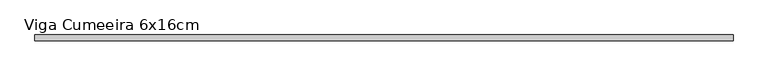
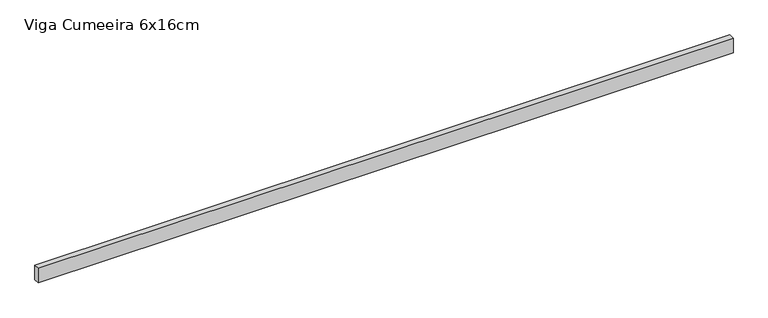
"""IFC4 building model written with IfcOpenShell, lengths in millimetres: beam geometry, Madeira de lei : Viga Cumeeira 6x16cm."""

import ifcopenshell
import ifcopenshell.guid

model = None  # the IFC model being written
_history = None  # IfcOwnerHistory: only IFC2X3 demands one
_inside = {}  # id of a spatial element -> (the spatial element, [elements in it])
_under = {}  # id of a project, library or spatial element -> (it, [spatial elements below it])
_declared = {}  # id of a project -> (the project, [libraries it declares])
_typed = {}  # id of a type object -> (the type object, [elements of that type])
_made_of = {}  # id of a material, layer set ... -> (it, [elements and type objects made of it])


def new_model(schema):
    """Start an empty IFC model of exactly this schema.

    Asked for "IFC4X3", IfcOpenShell would pick the latest addendum, in which some entities
    have other attributes; the version numbers below select the first issue.
    IFC2X3 requires an IfcOwnerHistory on every rooted entity: one is made here for all.
    """
    global model, _history
    if schema == "IFC4X3":
        model = ifcopenshell.file(schema_version=(4, 3, 0, 0))
    else:
        model = ifcopenshell.file(schema=schema)
    _inside.clear()
    _under.clear()
    _declared.clear()
    _typed.clear()
    _made_of.clear()
    _history = None
    if model.schema == "IFC2X3":
        org = make("IfcOrganization", Name="unknown")
        user = make(
            "IfcPersonAndOrganization",
            ThePerson=make("IfcPerson", FamilyName="unknown"),
            TheOrganization=org,
        )
        app = make(
            "IfcApplication",
            ApplicationDeveloper=org,
            Version="unknown",
            ApplicationFullName="unknown",
            ApplicationIdentifier="unknown",
        )
        _history = make(
            "IfcOwnerHistory",
            OwningUser=user,
            OwningApplication=app,
            ChangeAction="ADDED",
            CreationDate=0,
        )
    return model


def make(cls, **values):
    """One entity of the class cls with the attributes given. An attribute that is None is left unset."""
    return model.create_entity(
        cls, **{name: value for name, value in values.items() if value is not None}
    )


def rooted(cls, **values):
    """An entity with a GlobalId (a new one), such as an element, a storey or a relation."""
    return make(cls, GlobalId=ifcopenshell.guid.new(), OwnerHistory=_history, **values)


def si_unit(unit_type, name, prefix=None):
    """IfcSIUnit, for example si_unit("LENGTHUNIT", "METRE", prefix="MILLI")."""
    return make("IfcSIUnit", UnitType=unit_type, Prefix=prefix, Name=name)


def assignment(units):
    """IfcUnitAssignment: the units of a project."""
    return None if units is None else make("IfcUnitAssignment", Units=units)


def point(xyz):
    """IfcCartesianPoint."""
    return None if xyz is None else make("IfcCartesianPoint", Coordinates=xyz)


def direction(xyz):
    """IfcDirection."""
    return None if xyz is None else make("IfcDirection", DirectionRatios=xyz)


def frame(location, z_axis=None, x_axis=None):
    """IfcAxis2Placement3D, a coordinate frame: its origin and axes. An axis left out is left unset."""
    return make(
        "IfcAxis2Placement3D",
        Location=point(location),
        Axis=direction(z_axis),
        RefDirection=direction(x_axis),
    )


def origin():
    """The frame at (0, 0, 0) with its axes left unset."""
    return frame((0.0, 0.0, 0.0))


def place(relative_to, where):
    """IfcLocalPlacement: puts the frame where relative to a parent placement (None: the world)."""
    return make(
        "IfcLocalPlacement", PlacementRelTo=relative_to, RelativePlacement=where
    )


def context(
    kind, dimensions, precision=None, world=None, true_north=None, identifier=None
):
    """IfcGeometricRepresentationContext, for example the 3D "Model" context."""
    return make(
        "IfcGeometricRepresentationContext",
        ContextIdentifier=identifier,
        ContextType=kind,
        CoordinateSpaceDimension=dimensions,
        Precision=precision,
        WorldCoordinateSystem=world,
        TrueNorth=true_north,
    )


def project(units=None, contexts=None):
    """IfcProject with its units and contexts."""
    return rooted(
        "IfcProject",
        Name="project",
        RepresentationContexts=contexts,
        UnitsInContext=assignment(units),
    )


def spatial(cls, under=None, at=None, **own):
    """A site, building, storey or space (cls), placed at a placement, below another one or the project."""
    s = rooted(cls, ObjectPlacement=at, **own)
    if under is not None:
        _under.setdefault(under.id(), (under, []))[1].append(s)
    return s


def polyline(points):
    """IfcPolyline through the points."""
    return make("IfcPolyline", Points=[point(p) for p in points])


def outline(outer, holes=None, kind="AREA"):
    """IfcArbitraryClosedProfileDef: a profile drawn as a closed curve; with holes, ...WithVoids."""
    if holes is None:
        return make("IfcArbitraryClosedProfileDef", ProfileType=kind, OuterCurve=outer)
    return make(
        "IfcArbitraryProfileDefWithVoids",
        ProfileType=kind,
        OuterCurve=outer,
        InnerCurves=holes,
    )


def extrude(swept, where, along, depth):
    """IfcExtrudedAreaSolid: the profile swept, set in the frame where, extruded along a direction by depth."""
    return make(
        "IfcExtrudedAreaSolid",
        SweptArea=swept,
        Position=where,
        ExtrudedDirection=direction(along),
        Depth=depth,
    )


def shape(context_of_items, identifier, shape_type, items):
    """IfcShapeRepresentation: the items that make up one representation, for example the "Body"."""
    return make(
        "IfcShapeRepresentation",
        ContextOfItems=context_of_items,
        RepresentationIdentifier=identifier,
        RepresentationType=shape_type,
        Items=items,
    )


def source(mapping_origin, context_of_items, identifier, shape_type, items):
    """IfcRepresentationMap: a shape defined once, which mapped items show again and again."""
    return make(
        "IfcRepresentationMap",
        MappingOrigin=mapping_origin,
        MappedRepresentation=shape(context_of_items, identifier, shape_type, items),
    )


def transform(
    local_origin,
    x_axis=None,
    y_axis=None,
    z_axis=None,
    scale=None,
    scale2=None,
    scale3=None,
    uniform=True,
):
    """IfcCartesianTransformationOperator3D, or its non-uniform kind. x_axis, y_axis, z_axis: its Axis1, 2, 3."""
    if uniform:
        return make(
            "IfcCartesianTransformationOperator3D",
            Axis1=direction(x_axis),
            Axis2=direction(y_axis),
            LocalOrigin=point(local_origin),
            Scale=scale,
            Axis3=direction(z_axis),
        )
    return make(
        "IfcCartesianTransformationOperator3DnonUniform",
        Axis1=direction(x_axis),
        Axis2=direction(y_axis),
        LocalOrigin=point(local_origin),
        Scale=scale,
        Axis3=direction(z_axis),
        Scale2=scale2,
        Scale3=scale3,
    )


def mapped(mapping_source, mapping_target):
    """IfcMappedItem: shows the shape of a source again, moved by a transform."""
    return make(
        "IfcMappedItem", MappingSource=mapping_source, MappingTarget=mapping_target
    )


def made_of(thing, what):
    """Note that an element or type object is made of a material, layer set ...; save() writes the relation."""
    if what is not None:
        _made_of.setdefault(what.id(), (what, []))[1].append(thing)
    return thing


def element(
    cls,
    number,
    at=None,
    inside=None,
    cuts=None,
    type_object=None,
    material=None,
    context=None,
    identifier="Body",
    shape_type=None,
    held_by="IfcProductDefinitionShape",
    body=None,
    shapes=None,
    **own,
):
    """One element of the class cls, such as IfcWall. Its Tag is "e" and its number.

    at: its placement. inside: the storey or other place that contains it. cuts: it is an
    opening in that element (IfcRelVoidsElement). A single representation is given by context,
    identifier, shape_type and body (its items); several are given by shapes. held_by: the class
    of the entity that holds the representations. save() writes the other relations.
    """
    e = rooted(cls, Tag="e%d" % number, ObjectPlacement=at, **own)
    if body is not None:
        shapes = [shape(context, identifier, shape_type, body)]
    if shapes is not None:
        e.Representation = make(held_by, Representations=shapes)
    if inside is not None:
        _inside.setdefault(inside.id(), (inside, []))[1].append(e)
    if cuts is not None:
        rooted(
            "IfcRelVoidsElement", RelatingBuildingElement=cuts, RelatedOpeningElement=e
        )
    if type_object is not None:
        _typed.setdefault(type_object.id(), (type_object, []))[1].append(e)
    return made_of(e, material)


def aggregate(whole, parts):
    """IfcRelAggregates: a whole, such as a stair, and the parts it consists of."""
    return rooted("IfcRelAggregates", RelatingObject=whole, RelatedObjects=parts)


def save(model, path):
    """Write the relations noted so far, then the file.

    IfcRelAggregates (storeys below a building ...), IfcRelContainedInSpatialStructure (elements
    in a storey), IfcRelDefinesByType, IfcRelAssociatesMaterial and IfcRelDeclares: one each for
    every whole, place, type object, material and project.
    """
    for whole, parts in _under.values():
        aggregate(whole, parts)
    for where, things in _inside.values():
        rooted(
            "IfcRelContainedInSpatialStructure",
            RelatedElements=things,
            RelatingStructure=where,
        )
    for kind, things in _typed.values():
        rooted("IfcRelDefinesByType", RelatedObjects=things, RelatingType=kind)
    for what, things in _made_of.values():
        rooted("IfcRelAssociatesMaterial", RelatedObjects=things, RelatingMaterial=what)
    for by, libraries in _declared.values():
        rooted("IfcRelDeclares", RelatingContext=by, RelatedDefinitions=libraries)
    model.write(path)


def viga_cumeeira_6x16cm_d80f05ee(model_context):
    return source(origin(), model_context, "Body", "SweptSolid", [
        extrude(outline(polyline([(3626.5, 30.0), (3626.5, -30.0), (-3626.5, -30.0), (-3626.5, 30.0), (3626.5, 30.0)])), frame((0.0, 0.0, -80.0), z_axis=(0.0, 0.0, 1.0), x_axis=(1.0, 0.0, 0.0)), (0.0, 0.0, 1.0), 160.0),
    ])


if __name__ == "__main__":
    model = new_model("IFC4")
    model_context = context("Model", 3, world=origin())
    ifc_project = project(units=[si_unit("LENGTHUNIT", "METRE", prefix="MILLI")], contexts=[model_context])
    site = spatial("IfcSite", under=ifc_project)
    building = spatial("IfcBuilding", under=site)
    placement = place(None, origin())
    viga_cumeeira_6x16cm_shape = viga_cumeeira_6x16cm_d80f05ee(model_context)
    element("IfcBeam", 1, ObjectType="Madeira de lei : Viga Cumeeira 6x16cm", at=placement, inside=building, context=model_context, shape_type="MappedRepresentation", body=[
        mapped(viga_cumeeira_6x16cm_shape, transform((0.0, 0.0, 0.0), x_axis=(1.0, 0.0, 0.0), y_axis=(0.0, 1.0, 0.0), z_axis=(0.0, 0.0, 1.0))),
    ])
    save(model, "model.ifc")

# Revit data of these elements
# Type "Madeira de lei : Viga Cumeeira 6x16cm"
#   A = 0.02 m²
#   Length [instance default] = 1.524 m
#   b = 0.06 m
#   d = 0.16 m
#   Structural Material [instance default] = none
#   Assembly Code = ""
# Element 1 (IfcBeam, "Madeira de lei : Viga Cumeeira 6x16cm")
#   Structural Material = .MADEIRAMENTO
#   Materials on its faces: ".MADEIRAMENTO"
# Materials
#   ".MADEIRAMENTO": class ".CC_MADEIRAS", colour RGB 212 179 113, transparency 0, Cost = 0
